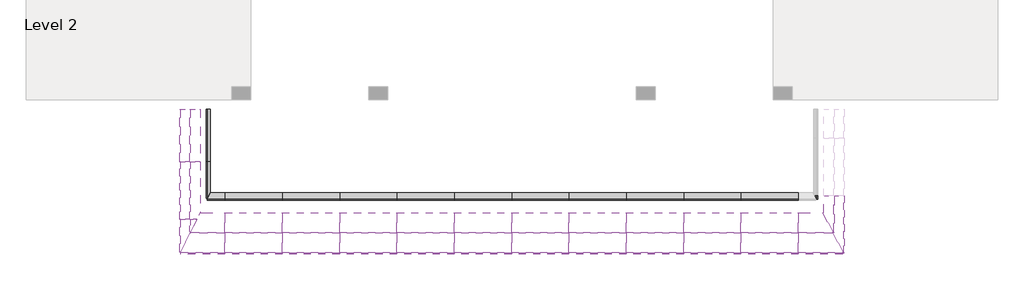
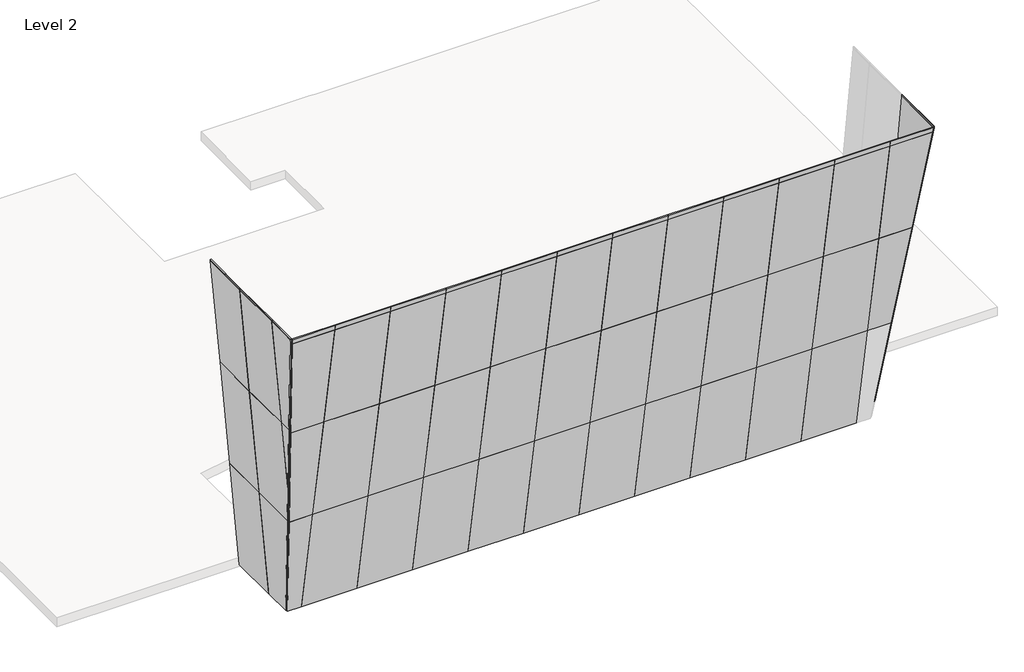
# One storey, part 1 of 2: 62 plates.
"""IFC4 building model written with IfcOpenShell, lengths in millimetres."""

import ifcopenshell
import ifcopenshell.guid

model = None  # the IFC model being written
_history = None  # IfcOwnerHistory: only IFC2X3 demands one
_inside = {}  # id of a spatial element -> (the spatial element, [elements in it])
_under = {}  # id of a project, library or spatial element -> (it, [spatial elements below it])
_declared = {}  # id of a project -> (the project, [libraries it declares])
_typed = {}  # id of a type object -> (the type object, [elements of that type])
_made_of = {}  # id of a material, layer set ... -> (it, [elements and type objects made of it])


def new_model(schema):
    """Start an empty IFC model of exactly this schema.

    Asked for "IFC4X3", IfcOpenShell would pick the latest addendum, in which some entities
    have other attributes; the version numbers below select the first issue.
    IFC2X3 requires an IfcOwnerHistory on every rooted entity: one is made here for all.
    """
    global model, _history
    if schema == "IFC4X3":
        model = ifcopenshell.file(schema_version=(4, 3, 0, 0))
    else:
        model = ifcopenshell.file(schema=schema)
    _inside.clear()
    _under.clear()
    _declared.clear()
    _typed.clear()
    _made_of.clear()
    _history = None
    if model.schema == "IFC2X3":
        org = make("IfcOrganization", Name="unknown")
        user = make(
            "IfcPersonAndOrganization",
            ThePerson=make("IfcPerson", FamilyName="unknown"),
            TheOrganization=org,
        )
        app = make(
            "IfcApplication",
            ApplicationDeveloper=org,
            Version="unknown",
            ApplicationFullName="unknown",
            ApplicationIdentifier="unknown",
        )
        _history = make(
            "IfcOwnerHistory",
            OwningUser=user,
            OwningApplication=app,
            ChangeAction="ADDED",
            CreationDate=0,
        )
    return model


def make(cls, **values):
    """One entity of the class cls with the attributes given. An attribute that is None is left unset."""
    return model.create_entity(
        cls, **{name: value for name, value in values.items() if value is not None}
    )


def rooted(cls, **values):
    """An entity with a GlobalId (a new one), such as an element, a storey or a relation."""
    return make(cls, GlobalId=ifcopenshell.guid.new(), OwnerHistory=_history, **values)


def si_unit(unit_type, name, prefix=None):
    """IfcSIUnit, for example si_unit("LENGTHUNIT", "METRE", prefix="MILLI")."""
    return make("IfcSIUnit", UnitType=unit_type, Prefix=prefix, Name=name)


def assignment(units):
    """IfcUnitAssignment: the units of a project."""
    return None if units is None else make("IfcUnitAssignment", Units=units)


def point(xyz):
    """IfcCartesianPoint."""
    return None if xyz is None else make("IfcCartesianPoint", Coordinates=xyz)


def direction(xyz):
    """IfcDirection."""
    return None if xyz is None else make("IfcDirection", DirectionRatios=xyz)


def frame(location, z_axis=None, x_axis=None):
    """IfcAxis2Placement3D, a coordinate frame: its origin and axes. An axis left out is left unset."""
    return make(
        "IfcAxis2Placement3D",
        Location=point(location),
        Axis=direction(z_axis),
        RefDirection=direction(x_axis),
    )


def origin():
    """The frame at (0, 0, 0) with its axes left unset."""
    return frame((0.0, 0.0, 0.0))


def origin_with_axes():
    """The frame at (0, 0, 0) with the z axis (0, 0, 1) and the x axis (1, 0, 0) written out."""
    return frame((0.0, 0.0, 0.0), z_axis=(0.0, 0.0, 1.0), x_axis=(1.0, 0.0, 0.0))


def place(relative_to, where):
    """IfcLocalPlacement: puts the frame where relative to a parent placement (None: the world)."""
    return make(
        "IfcLocalPlacement", PlacementRelTo=relative_to, RelativePlacement=where
    )


def context(
    kind, dimensions, precision=None, world=None, true_north=None, identifier=None
):
    """IfcGeometricRepresentationContext, for example the 3D "Model" context."""
    return make(
        "IfcGeometricRepresentationContext",
        ContextIdentifier=identifier,
        ContextType=kind,
        CoordinateSpaceDimension=dimensions,
        Precision=precision,
        WorldCoordinateSystem=world,
        TrueNorth=true_north,
    )


def project(units=None, contexts=None):
    """IfcProject with its units and contexts."""
    return rooted(
        "IfcProject",
        Name="project",
        RepresentationContexts=contexts,
        UnitsInContext=assignment(units),
    )


def spatial(cls, under=None, at=None, **own):
    """A site, building, storey or space (cls), placed at a placement, below another one or the project."""
    s = rooted(cls, ObjectPlacement=at, **own)
    if under is not None:
        _under.setdefault(under.id(), (under, []))[1].append(s)
    return s


def polyline(points):
    """IfcPolyline through the points."""
    return make("IfcPolyline", Points=[point(p) for p in points])


def outline(outer, holes=None, kind="AREA"):
    """IfcArbitraryClosedProfileDef: a profile drawn as a closed curve; with holes, ...WithVoids."""
    if holes is None:
        return make("IfcArbitraryClosedProfileDef", ProfileType=kind, OuterCurve=outer)
    return make(
        "IfcArbitraryProfileDefWithVoids",
        ProfileType=kind,
        OuterCurve=outer,
        InnerCurves=holes,
    )


def extrude(swept, where, along, depth):
    """IfcExtrudedAreaSolid: the profile swept, set in the frame where, extruded along a direction by depth."""
    return make(
        "IfcExtrudedAreaSolid",
        SweptArea=swept,
        Position=where,
        ExtrudedDirection=direction(along),
        Depth=depth,
    )


def shape(context_of_items, identifier, shape_type, items):
    """IfcShapeRepresentation: the items that make up one representation, for example the "Body"."""
    return make(
        "IfcShapeRepresentation",
        ContextOfItems=context_of_items,
        RepresentationIdentifier=identifier,
        RepresentationType=shape_type,
        Items=items,
    )


def source(mapping_origin, context_of_items, identifier, shape_type, items):
    """IfcRepresentationMap: a shape defined once, which mapped items show again and again."""
    return make(
        "IfcRepresentationMap",
        MappingOrigin=mapping_origin,
        MappedRepresentation=shape(context_of_items, identifier, shape_type, items),
    )


def transform(
    local_origin,
    x_axis=None,
    y_axis=None,
    z_axis=None,
    scale=None,
    scale2=None,
    scale3=None,
    uniform=True,
):
    """IfcCartesianTransformationOperator3D, or its non-uniform kind. x_axis, y_axis, z_axis: its Axis1, 2, 3."""
    if uniform:
        return make(
            "IfcCartesianTransformationOperator3D",
            Axis1=direction(x_axis),
            Axis2=direction(y_axis),
            LocalOrigin=point(local_origin),
            Scale=scale,
            Axis3=direction(z_axis),
        )
    return make(
        "IfcCartesianTransformationOperator3DnonUniform",
        Axis1=direction(x_axis),
        Axis2=direction(y_axis),
        LocalOrigin=point(local_origin),
        Scale=scale,
        Axis3=direction(z_axis),
        Scale2=scale2,
        Scale3=scale3,
    )


def mapped(mapping_source, mapping_target):
    """IfcMappedItem: shows the shape of a source again, moved by a transform."""
    return make(
        "IfcMappedItem", MappingSource=mapping_source, MappingTarget=mapping_target
    )


def made_of(thing, what):
    """Note that an element or type object is made of a material, layer set ...; save() writes the relation."""
    if what is not None:
        _made_of.setdefault(what.id(), (what, []))[1].append(thing)
    return thing


def element(
    cls,
    number,
    at=None,
    inside=None,
    cuts=None,
    type_object=None,
    material=None,
    context=None,
    identifier="Body",
    shape_type=None,
    held_by="IfcProductDefinitionShape",
    body=None,
    shapes=None,
    **own,
):
    """One element of the class cls, such as IfcWall. Its Tag is "e" and its number.

    at: its placement. inside: the storey or other place that contains it. cuts: it is an
    opening in that element (IfcRelVoidsElement). A single representation is given by context,
    identifier, shape_type and body (its items); several are given by shapes. held_by: the class
    of the entity that holds the representations. save() writes the other relations.
    """
    e = rooted(cls, Tag="e%d" % number, ObjectPlacement=at, **own)
    if body is not None:
        shapes = [shape(context, identifier, shape_type, body)]
    if shapes is not None:
        e.Representation = make(held_by, Representations=shapes)
    if inside is not None:
        _inside.setdefault(inside.id(), (inside, []))[1].append(e)
    if cuts is not None:
        rooted(
            "IfcRelVoidsElement", RelatingBuildingElement=cuts, RelatedOpeningElement=e
        )
    if type_object is not None:
        _typed.setdefault(type_object.id(), (type_object, []))[1].append(e)
    return made_of(e, material)


def aggregate(whole, parts):
    """IfcRelAggregates: a whole, such as a stair, and the parts it consists of."""
    return rooted("IfcRelAggregates", RelatingObject=whole, RelatedObjects=parts)


def save(model, path):
    """Write the relations noted so far, then the file.

    IfcRelAggregates (storeys below a building ...), IfcRelContainedInSpatialStructure (elements
    in a storey), IfcRelDefinesByType, IfcRelAssociatesMaterial and IfcRelDeclares: one each for
    every whole, place, type object, material and project.
    """
    for whole, parts in _under.values():
        aggregate(whole, parts)
    for where, things in _inside.values():
        rooted(
            "IfcRelContainedInSpatialStructure",
            RelatedElements=things,
            RelatingStructure=where,
        )
    for kind, things in _typed.values():
        rooted("IfcRelDefinesByType", RelatedObjects=things, RelatingType=kind)
    for what, things in _made_of.values():
        rooted("IfcRelAssociatesMaterial", RelatedObjects=things, RelatingMaterial=what)
    for by, libraries in _declared.values():
        rooted("IfcRelDeclares", RelatingContext=by, RelatedDefinitions=libraries)
    model.write(path)


def system_panel_glazed_2e91cb65(model_context):
    return source(origin(), model_context, "Body", "SweptSolid", [
        extrude(outline(polyline([(838.2000002, -44.45), (-838.2000002, -44.45), (-838.2000002, -19.05), (838.2000002, -19.05), (838.2000002, -44.45)])), origin_with_axes(), (0.0, 0.0, 1.0), 3657.6),
    ])


def system_panel_glazed_41c8569a(model_context):
    return source(origin(), model_context, "Body", "SweptSolid", [
        extrude(outline(polyline([(3054.1438606, -268.2393521), (0.0, 268.2393521), (3054.1438606, 268.2393521), (3054.1438606, -268.2393521)])), frame((0.0, -44.45, 0.0), z_axis=(0.0, 1.0, 0.0), x_axis=(0.0, 0.0, 1.0)), (0.0, 0.0, 1.0), 25.4),
    ])


def system_panel_glazed_2bad594a(model_context):
    return source(origin(), model_context, "Body", "SweptSolid", [
        extrude(outline(polyline([(0.0, -797.3917397), (0.0, 154.912342), (3657.6, 797.3917397), (3657.6, -797.3917397), (0.0, -797.3917397)])), frame((0.0, -44.45, 0.0), z_axis=(0.0, 1.0, 0.0), x_axis=(0.0, 0.0, 1.0)), (0.0, 0.0, 1.0), 25.4),
    ])


def system_panel_glazed_87679f4c(model_context):
    return source(origin(), model_context, "Body", "SweptSolid", [
        extrude(outline(polyline([(0.0, -914.4), (0.0, 680.3834794), (1332.2432262, 914.4), (3657.6, 914.4), (3657.6, -914.4), (0.0, -914.4)])), frame((0.0, -44.45, 0.0), z_axis=(0.0, 1.0, 0.0), x_axis=(0.0, 0.0, 1.0)), (0.0, 0.0, 1.0), 25.4),
    ])


def system_panel_glazed_96c5221b(model_context):
    return source(origin(), model_context, "Body", "SweptSolid", [
        extrude(outline(polyline([(0.0, -204.2314386), (2325.3567738, 204.2314386), (2325.3567738, -204.2314386), (0.0, -204.2314386)])), frame((0.0, -44.45, 0.0), z_axis=(0.0, 1.0, 0.0), x_axis=(0.0, 0.0, 1.0)), (0.0, 0.0, 1.0), 25.4),
    ])


def system_panel_glazed_1f34555f(model_context):
    return source(origin(), model_context, "Body", "SweptSolid", [
        extrude(outline(polyline([(914.4, -44.45), (-914.4, -44.45), (-914.4, -19.05), (914.4, -19.05), (914.4, -44.45)])), origin_with_axes(), (0.0, 0.0, 1.0), 3657.6),
    ])


def system_panel_glazed_ce152239(model_context):
    return source(origin(), model_context, "Body", "SweptSolid", [
        extrude(outline(polyline([(0.0, -525.4711374), (0.0, -117.0082603), (3657.6, 525.4711374), (3657.6, -525.4711374), (0.0, -525.4711374)])), frame((0.0, -44.45, 0.0), z_axis=(0.0, 1.0, 0.0), x_axis=(0.0, 0.0, 1.0)), (0.0, 0.0, 1.0), 25.4),
    ])


def system_panel_glazed_8b4ddac8(model_context):
    return source(origin(), model_context, "Body", "SweptSolid", [
        extrude(outline(polyline([(838.2000002, -44.45), (-838.2000002, -44.45), (-838.2000002, -19.05), (838.2000002, -19.05), (838.2000002, -44.45)])), origin_with_axes(), (0.0, 0.0, 1.0), 41.9143134),
    ])


def system_panel_glazed_7f82afe2(model_context):
    return source(origin(), model_context, "Body", "SweptSolid", [
        extrude(outline(polyline([(914.4, -44.45), (-914.4, -44.45), (-914.4, -19.05), (914.4, -19.05), (914.4, -44.45)])), origin_with_axes(), (0.0, 0.0, 1.0), 41.9143134),
    ])


def system_panel_glazed_3146f186(model_context):
    return source(origin(), model_context, "Body", "SweptSolid", [
        extrude(outline(polyline([(0.0, -529.1523878), (0.0, 521.789887), (41.9143134, 529.1523878), (41.9143134, -529.1523878), (0.0, -529.1523878)])), frame((0.0, -44.45, 0.0), z_axis=(0.0, 1.0, 0.0), x_axis=(0.0, 0.0, 1.0)), (0.0, 0.0, 1.0), 25.4),
    ])


def system_panel_glazed_f4345ae3(model_context):
    return source(origin(), model_context, "Body", "SweptSolid", [
        extrude(outline(polyline([(914.4, -44.45), (-914.4, -44.45), (-914.4, -19.05), (914.4, -19.05), (914.4, -44.45)])), origin_with_axes(), (0.0, 0.0, 1.0), 169.2731269),
    ])


def system_panel_glazed_bcd6892e(model_context):
    return source(origin(), model_context, "Body", "SweptSolid", [
        extrude(outline(polyline([(0.0, 53.0003468), (0.0, 589.4790509), (3657.6, 589.4790509), (3657.6, -589.4790509), (0.0, 53.0003468)])), frame((0.0, -44.45, 0.0), z_axis=(0.0, 1.0, 0.0), x_axis=(0.0, 0.0, 1.0)), (0.0, 0.0, 1.0), 25.4),
    ])


def system_panel_glazed_e7bd2299(model_context):
    return source(origin(), model_context, "Body", "SweptSolid", [
        extrude(outline(polyline([(0.0, -268.2393521), (0.0, 910.7187498), (3657.6, 910.7187498), (3657.6, -910.7187498), (0.0, -268.2393521)])), frame((0.0, -44.45, 0.0), z_axis=(0.0, 1.0, 0.0), x_axis=(0.0, 0.0, 1.0)), (0.0, 0.0, 1.0), 25.4),
    ])


def system_panel_glazed_0a43eb3e(model_context):
    return source(origin(), model_context, "Body", "SweptSolid", [
        extrude(outline(polyline([(0.0, -907.0374994), (0.0, 914.4000002), (41.9143134, 914.4000002), (41.9143134, -914.4000002), (0.0, -907.0374994)])), frame((0.0, -44.45, 0.0), z_axis=(0.0, 1.0, 0.0), x_axis=(0.0, 0.0, 1.0)), (0.0, 0.0, 1.0), 25.4),
    ])


def system_panel_glazed_35afb83b(model_context):
    return source(origin(), model_context, "Body", "SweptSolid", [
        extrude(outline(polyline([(0.0, -71.0314805), (0.0, 386.1685195), (3657.6, 386.1685195), (3657.6, -386.1685195), (0.0, -71.0314805)])), frame((0.0, -44.45, 0.0), z_axis=(0.0, 1.0, 0.0), x_axis=(0.0, 0.0, 1.0)), (0.0, 0.0, 1.0), 25.4),
    ])


def system_panel_glazed_d5b9b34d(model_context):
    return source(origin(), model_context, "Body", "SweptSolid", [
        extrude(outline(polyline([(0.0, -228.6), (0.0, 543.7370389), (3657.6, 543.7370389), (3657.6, -543.7370389), (0.0, -228.6)])), frame((0.0, -44.45, 0.0), z_axis=(0.0, 1.0, 0.0), x_axis=(0.0, 0.0, 1.0)), (0.0, 0.0, 1.0), 25.4),
    ])


def system_panel_glazed_127879aa(model_context):
    return source(origin(), model_context, "Body", "SweptSolid", [
        extrude(outline(polyline([(0.0, -543.7370389), (0.0, 228.6), (3657.6, 543.7370389), (3657.6, -543.7370389), (0.0, -543.7370389)])), frame((0.0, -44.45, 0.0), z_axis=(0.0, 1.0, 0.0), x_axis=(0.0, 0.0, 1.0)), (0.0, 0.0, 1.0), 25.4),
    ])


def system_panel_glazed_cde5e94a(model_context):
    return source(origin(), model_context, "Body", "SweptSolid", [
        extrude(outline(polyline([(0.0, -386.1685195), (0.0, 701.3055584), (3657.6, 701.3055584), (3657.6, -701.3055584), (0.0, -386.1685195)])), frame((0.0, -44.45, 0.0), z_axis=(0.0, 1.0, 0.0), x_axis=(0.0, 0.0, 1.0)), (0.0, 0.0, 1.0), 25.4),
    ])


def system_panel_glazed_b3fa7013(model_context):
    return source(origin(), model_context, "Body", "SweptSolid", [
        extrude(outline(polyline([(0.0, -701.3055584), (0.0, 386.1685195), (3657.6, 701.3055584), (3657.6, -701.3055584), (0.0, -701.3055584)])), frame((0.0, -44.45, 0.0), z_axis=(0.0, 1.0, 0.0), x_axis=(0.0, 0.0, 1.0)), (0.0, 0.0, 1.0), 25.4),
    ])


def system_panel_glazed_d86b06c2(model_context):
    return source(origin(), model_context, "Body", "SweptSolid", [
        extrude(outline(polyline([(0.0, -694.0133132), (0.0, 708.5978036), (169.2731269, 708.5978036), (169.2731269, -708.5978036), (0.0, -694.0133132)])), frame((0.0, -44.45, 0.0), z_axis=(0.0, 1.0, 0.0), x_axis=(0.0, 0.0, 1.0)), (0.0, 0.0, 1.0), 25.4),
    ])


def system_panel_glazed_9c30f1a4(model_context):
    return source(origin(), model_context, "Body", "SweptSolid", [
        extrude(outline(polyline([(0.0, -708.5978036), (0.0, 694.0133132), (169.2731269, 708.5978036), (169.2731269, -708.5978036), (0.0, -708.5978036)])), frame((0.0, -44.45, 0.0), z_axis=(0.0, 1.0, 0.0), x_axis=(0.0, 0.0, 1.0)), (0.0, 0.0, 1.0), 25.4),
    ])


model = new_model("IFC4")

# Units and contexts
model_context = context("Model", 3, world=origin())
ifc_project = project(units=[si_unit("LENGTHUNIT", "METRE", prefix="MILLI")], contexts=[model_context])

# Site, building, storey
site = spatial("IfcSite", under=ifc_project)
building = spatial("IfcBuilding", under=site)
storey = spatial("IfcBuildingStorey", under=building, Name="Level 2", Elevation=3657.6)

# Plates
placement = place(None, origin())
system_panel_glazed_shape = system_panel_glazed_2e91cb65(model_context)
element("IfcPlate", 1, ObjectType="System Panel : Glazed", at=placement, inside=storey, context=model_context, shape_type="MappedRepresentation", body=[
    mapped(system_panel_glazed_shape, transform((-10766.9154339, -10749.0984697, 3656.4931221), x_axis=(0.0, -1.0, 0.0), y_axis=(0.9961946980917455, 0.0, 0.08715574274765803), z_axis=(-0.08715574274765803, 0.0, 0.9961946980917455))),
])
element("IfcPlate", 2, ObjectType="System Panel : Glazed", at=placement, inside=storey, context=model_context, shape_type="MappedRepresentation", body=[
    mapped(system_panel_glazed_shape, transform((-11085.6962786, -10749.0984697, 7300.1748498), x_axis=(0.0, -1.0, 0.0), y_axis=(0.9961946980917455, 0.0, 0.08715574274765803), z_axis=(-0.08715574274765803, 0.0, 0.9961946980917455))),
])
element("IfcPlate", 3, ObjectType="System Panel : Glazed", at=placement, inside=storey, context=model_context, shape_type="MappedRepresentation", body=[
    mapped(system_panel_glazed_shape, transform((-11404.4771233, -10749.0984697, 10943.8565775), x_axis=(0.0, -1.0, 0.0), y_axis=(0.9961946980917455, 0.0, 0.08715574274765803), z_axis=(-0.08715574274765803, 0.0, 0.9961946980917455))),
])
system_panel_glazed_2_shape = system_panel_glazed_41c8569a(model_context)
element("IfcPlate", 4, ObjectType="System Panel : Glazed", at=placement, inside=storey, context=model_context, shape_type="MappedRepresentation", body=[
    mapped(system_panel_glazed_2_shape, transform((8487.8855556, -12939.6344332, 4257.6529286), x_axis=(0.0, 1.0, 0.0), y_axis=(-0.9961946980917455, 0.0, 0.08715574274765803), z_axis=(0.08715574274765803, 0.0, 0.9961946980917455))),
])
system_panel_glazed_3_shape = system_panel_glazed_2bad594a(model_context)
element("IfcPlate", 5, ObjectType="System Panel : Glazed", at=placement, inside=storey, context=model_context, shape_type="MappedRepresentation", body=[
    mapped(system_panel_glazed_3_shape, transform((-10766.9154339, -12384.6902096, 3656.4931221), x_axis=(0.0, -1.0, 0.0), y_axis=(0.9961946980917455, 0.0, 0.08715574274765803), z_axis=(-0.08715574274765803, 0.0, 0.9961946980917455))),
])
system_panel_glazed_4_shape = system_panel_glazed_87679f4c(model_context)
element("IfcPlate", 6, ObjectType="System Panel : Glazed", at=placement, inside=storey, context=model_context, shape_type="MappedRepresentation", body=[
    mapped(system_panel_glazed_4_shape, transform((-11085.6962786, -12501.6984699, 7300.1748498), x_axis=(0.0, -1.0, 0.0), y_axis=(0.9961946980917455, 0.0, 0.08715574274765803), z_axis=(-0.08715574274765803, 0.0, 0.9961946980917455))),
])
system_panel_glazed_5_shape = system_panel_glazed_96c5221b(model_context)
element("IfcPlate", 7, ObjectType="System Panel : Glazed", at=placement, inside=storey, context=model_context, shape_type="MappedRepresentation", body=[
    mapped(system_panel_glazed_5_shape, transform((-11201.8089265, -13620.3299085, 8627.3484884), x_axis=(0.0, -1.0, 0.0), y_axis=(0.9961946980917455, 0.0, 0.08715574274765803), z_axis=(-0.08715574274765803, 0.0, 0.9961946980917455))),
])
system_panel_glazed_6_shape = system_panel_glazed_1f34555f(model_context)
element("IfcPlate", 8, ObjectType="System Panel : Glazed", at=placement, inside=storey, context=model_context, shape_type="MappedRepresentation", body=[
    mapped(system_panel_glazed_6_shape, transform((-11404.4771233, -12501.6984699, 10943.8565775), x_axis=(0.0, -1.0, 0.0), y_axis=(0.9961946980917455, 0.0, 0.08715574274765803), z_axis=(-0.08715574274765803, 0.0, 0.9961946980917455))),
])
element("IfcPlate", 9, ObjectType="System Panel : Glazed", at=placement, inside=storey, context=model_context, shape_type="MappedRepresentation", body=[
    mapped(system_panel_glazed_6_shape, transform((-9408.1607851, -12552.1096101, 3655.3946681), x_axis=(1.0, 0.0, 0.0), y_axis=(0.0, 0.9848077530122081, 0.17364817766693014), z_axis=(0.0, -0.17364817766693014, 0.9848077530122081))),
])
element("IfcPlate", 10, ObjectType="System Panel : Glazed", at=placement, inside=storey, context=model_context, shape_type="MappedRepresentation", body=[
    mapped(system_panel_glazed_6_shape, transform((-7579.3607851, -12552.1096101, 3655.3946681), x_axis=(1.0, 0.0, 0.0), y_axis=(0.0, 0.9848077530122081, 0.17364817766693014), z_axis=(0.0, -0.17364817766693014, 0.9848077530122081))),
])
element("IfcPlate", 11, ObjectType="System Panel : Glazed", at=placement, inside=storey, context=model_context, shape_type="MappedRepresentation", body=[
    mapped(system_panel_glazed_6_shape, transform((-5750.5607851, -12552.1096101, 3655.3946681), x_axis=(1.0, 0.0, 0.0), y_axis=(0.0, 0.9848077530122081, 0.17364817766693014), z_axis=(0.0, -0.17364817766693014, 0.9848077530122081))),
])
element("IfcPlate", 12, ObjectType="System Panel : Glazed", at=placement, inside=storey, context=model_context, shape_type="MappedRepresentation", body=[
    mapped(system_panel_glazed_6_shape, transform((-3921.7607851, -12552.1096101, 3655.3946681), x_axis=(1.0, 0.0, 0.0), y_axis=(0.0, 0.9848077530122081, 0.17364817766693014), z_axis=(0.0, -0.17364817766693014, 0.9848077530122081))),
])
element("IfcPlate", 13, ObjectType="System Panel : Glazed", at=placement, inside=storey, context=model_context, shape_type="MappedRepresentation", body=[
    mapped(system_panel_glazed_6_shape, transform((-2092.9607851, -12552.1096101, 3655.3946681), x_axis=(1.0, 0.0, 0.0), y_axis=(0.0, 0.9848077530122081, 0.17364817766693014), z_axis=(0.0, -0.17364817766693014, 0.9848077530122081))),
])
element("IfcPlate", 14, ObjectType="System Panel : Glazed", at=placement, inside=storey, context=model_context, shape_type="MappedRepresentation", body=[
    mapped(system_panel_glazed_6_shape, transform((-264.1607851, -12552.1096101, 3655.3946681), x_axis=(1.0, 0.0, 0.0), y_axis=(0.0, 0.9848077530122081, 0.17364817766693014), z_axis=(0.0, -0.17364817766693014, 0.9848077530122081))),
])
element("IfcPlate", 15, ObjectType="System Panel : Glazed", at=placement, inside=storey, context=model_context, shape_type="MappedRepresentation", body=[
    mapped(system_panel_glazed_6_shape, transform((1564.6392149, -12552.1096101, 3655.3946681), x_axis=(1.0, 0.0, 0.0), y_axis=(0.0, 0.9848077530122081, 0.17364817766693014), z_axis=(0.0, -0.17364817766693014, 0.9848077530122081))),
])
element("IfcPlate", 16, ObjectType="System Panel : Glazed", at=placement, inside=storey, context=model_context, shape_type="MappedRepresentation", body=[
    mapped(system_panel_glazed_6_shape, transform((3393.4392149, -12552.1096101, 3655.3946681), x_axis=(1.0, 0.0, 0.0), y_axis=(0.0, 0.9848077530122081, 0.17364817766693014), z_axis=(0.0, -0.17364817766693014, 0.9848077530122081))),
])
element("IfcPlate", 17, ObjectType="System Panel : Glazed", at=placement, inside=storey, context=model_context, shape_type="MappedRepresentation", body=[
    mapped(system_panel_glazed_6_shape, transform((5222.2392149, -12552.1096101, 3655.3946681), x_axis=(1.0, 0.0, 0.0), y_axis=(0.0, 0.9848077530122081, 0.17364817766693014), z_axis=(0.0, -0.17364817766693014, 0.9848077530122081))),
])
element("IfcPlate", 18, ObjectType="System Panel : Glazed", at=placement, inside=storey, context=model_context, shape_type="MappedRepresentation", body=[
    mapped(system_panel_glazed_6_shape, transform((7051.0392149, -12552.1096101, 3655.3946681), x_axis=(1.0, 0.0, 0.0), y_axis=(0.0, 0.9848077530122081, 0.17364817766693014), z_axis=(0.0, -0.17364817766693014, 0.9848077530122081))),
])
element("IfcPlate", 19, ObjectType="System Panel : Glazed", at=placement, inside=storey, context=model_context, shape_type="MappedRepresentation", body=[
    mapped(system_panel_glazed_6_shape, transform((-9408.1607851, -13187.2451847, 7257.4275056), x_axis=(1.0, 0.0, 0.0), y_axis=(0.0, 0.9848077530122081, 0.17364817766693014), z_axis=(0.0, -0.17364817766693014, 0.9848077530122081))),
])
element("IfcPlate", 20, ObjectType="System Panel : Glazed", at=placement, inside=storey, context=model_context, shape_type="MappedRepresentation", body=[
    mapped(system_panel_glazed_6_shape, transform((-7579.3607851, -13187.2451847, 7257.4275056), x_axis=(1.0, 0.0, 0.0), y_axis=(0.0, 0.9848077530122081, 0.17364817766693014), z_axis=(0.0, -0.17364817766693014, 0.9848077530122081))),
])
element("IfcPlate", 21, ObjectType="System Panel : Glazed", at=placement, inside=storey, context=model_context, shape_type="MappedRepresentation", body=[
    mapped(system_panel_glazed_6_shape, transform((-5750.5607851, -13187.2451847, 7257.4275056), x_axis=(1.0, 0.0, 0.0), y_axis=(0.0, 0.9848077530122081, 0.17364817766693014), z_axis=(0.0, -0.17364817766693014, 0.9848077530122081))),
])
element("IfcPlate", 22, ObjectType="System Panel : Glazed", at=placement, inside=storey, context=model_context, shape_type="MappedRepresentation", body=[
    mapped(system_panel_glazed_6_shape, transform((-3921.7607851, -13187.2451847, 7257.4275056), x_axis=(1.0, 0.0, 0.0), y_axis=(0.0, 0.9848077530122081, 0.17364817766693014), z_axis=(0.0, -0.17364817766693014, 0.9848077530122081))),
])
element("IfcPlate", 23, ObjectType="System Panel : Glazed", at=placement, inside=storey, context=model_context, shape_type="MappedRepresentation", body=[
    mapped(system_panel_glazed_6_shape, transform((-2092.9607851, -13187.2451847, 7257.4275056), x_axis=(1.0, 0.0, 0.0), y_axis=(0.0, 0.9848077530122081, 0.17364817766693014), z_axis=(0.0, -0.17364817766693014, 0.9848077530122081))),
])
element("IfcPlate", 24, ObjectType="System Panel : Glazed", at=placement, inside=storey, context=model_context, shape_type="MappedRepresentation", body=[
    mapped(system_panel_glazed_6_shape, transform((-264.1607851, -13187.2451847, 7257.4275056), x_axis=(1.0, 0.0, 0.0), y_axis=(0.0, 0.9848077530122081, 0.17364817766693014), z_axis=(0.0, -0.17364817766693014, 0.9848077530122081))),
])
element("IfcPlate", 25, ObjectType="System Panel : Glazed", at=placement, inside=storey, context=model_context, shape_type="MappedRepresentation", body=[
    mapped(system_panel_glazed_6_shape, transform((1564.6392149, -13187.2451847, 7257.4275056), x_axis=(1.0, 0.0, 0.0), y_axis=(0.0, 0.9848077530122081, 0.17364817766693014), z_axis=(0.0, -0.17364817766693014, 0.9848077530122081))),
])
element("IfcPlate", 26, ObjectType="System Panel : Glazed", at=placement, inside=storey, context=model_context, shape_type="MappedRepresentation", body=[
    mapped(system_panel_glazed_6_shape, transform((3393.4392149, -13187.2451847, 7257.4275056), x_axis=(1.0, 0.0, 0.0), y_axis=(0.0, 0.9848077530122081, 0.17364817766693014), z_axis=(0.0, -0.17364817766693014, 0.9848077530122081))),
])
element("IfcPlate", 27, ObjectType="System Panel : Glazed", at=placement, inside=storey, context=model_context, shape_type="MappedRepresentation", body=[
    mapped(system_panel_glazed_6_shape, transform((5222.2392149, -13187.2451847, 7257.4275056), x_axis=(1.0, 0.0, 0.0), y_axis=(0.0, 0.9848077530122081, 0.17364817766693014), z_axis=(0.0, -0.17364817766693014, 0.9848077530122081))),
])
element("IfcPlate", 28, ObjectType="System Panel : Glazed", at=placement, inside=storey, context=model_context, shape_type="MappedRepresentation", body=[
    mapped(system_panel_glazed_6_shape, transform((7051.0392149, -13187.2451847, 7257.4275056), x_axis=(1.0, 0.0, 0.0), y_axis=(0.0, 0.9848077530122081, 0.17364817766693014), z_axis=(0.0, -0.17364817766693014, 0.9848077530122081))),
])
element("IfcPlate", 29, ObjectType="System Panel : Glazed", at=placement, inside=storey, context=model_context, shape_type="MappedRepresentation", body=[
    mapped(system_panel_glazed_6_shape, transform((-9408.1607851, -13822.3807593, 10859.460343), x_axis=(1.0, 0.0, 0.0), y_axis=(0.0, 0.9848077530122081, 0.17364817766693014), z_axis=(0.0, -0.17364817766693014, 0.9848077530122081))),
])
element("IfcPlate", 30, ObjectType="System Panel : Glazed", at=placement, inside=storey, context=model_context, shape_type="MappedRepresentation", body=[
    mapped(system_panel_glazed_6_shape, transform((-7579.3607851, -13822.3807593, 10859.460343), x_axis=(1.0, 0.0, 0.0), y_axis=(0.0, 0.9848077530122081, 0.17364817766693014), z_axis=(0.0, -0.17364817766693014, 0.9848077530122081))),
])
element("IfcPlate", 31, ObjectType="System Panel : Glazed", at=placement, inside=storey, context=model_context, shape_type="MappedRepresentation", body=[
    mapped(system_panel_glazed_6_shape, transform((-5750.5607851, -13822.3807593, 10859.460343), x_axis=(1.0, 0.0, 0.0), y_axis=(0.0, 0.9848077530122081, 0.17364817766693014), z_axis=(0.0, -0.17364817766693014, 0.9848077530122081))),
])
element("IfcPlate", 32, ObjectType="System Panel : Glazed", at=placement, inside=storey, context=model_context, shape_type="MappedRepresentation", body=[
    mapped(system_panel_glazed_6_shape, transform((-3921.7607851, -13822.3807593, 10859.460343), x_axis=(1.0, 0.0, 0.0), y_axis=(0.0, 0.9848077530122081, 0.17364817766693014), z_axis=(0.0, -0.17364817766693014, 0.9848077530122081))),
])
element("IfcPlate", 33, ObjectType="System Panel : Glazed", at=placement, inside=storey, context=model_context, shape_type="MappedRepresentation", body=[
    mapped(system_panel_glazed_6_shape, transform((-2092.9607851, -13822.3807593, 10859.460343), x_axis=(1.0, 0.0, 0.0), y_axis=(0.0, 0.9848077530122081, 0.17364817766693014), z_axis=(0.0, -0.17364817766693014, 0.9848077530122081))),
])
element("IfcPlate", 34, ObjectType="System Panel : Glazed", at=placement, inside=storey, context=model_context, shape_type="MappedRepresentation", body=[
    mapped(system_panel_glazed_6_shape, transform((-264.1607851, -13822.3807593, 10859.460343), x_axis=(1.0, 0.0, 0.0), y_axis=(0.0, 0.9848077530122081, 0.17364817766693014), z_axis=(0.0, -0.17364817766693014, 0.9848077530122081))),
])
element("IfcPlate", 35, ObjectType="System Panel : Glazed", at=placement, inside=storey, context=model_context, shape_type="MappedRepresentation", body=[
    mapped(system_panel_glazed_6_shape, transform((1564.6392149, -13822.3807593, 10859.460343), x_axis=(1.0, 0.0, 0.0), y_axis=(0.0, 0.9848077530122081, 0.17364817766693014), z_axis=(0.0, -0.17364817766693014, 0.9848077530122081))),
])
element("IfcPlate", 36, ObjectType="System Panel : Glazed", at=placement, inside=storey, context=model_context, shape_type="MappedRepresentation", body=[
    mapped(system_panel_glazed_6_shape, transform((3393.4392149, -13822.3807593, 10859.460343), x_axis=(1.0, 0.0, 0.0), y_axis=(0.0, 0.9848077530122081, 0.17364817766693014), z_axis=(0.0, -0.17364817766693014, 0.9848077530122081))),
])
element("IfcPlate", 37, ObjectType="System Panel : Glazed", at=placement, inside=storey, context=model_context, shape_type="MappedRepresentation", body=[
    mapped(system_panel_glazed_6_shape, transform((5222.2392149, -13822.3807593, 10859.460343), x_axis=(1.0, 0.0, 0.0), y_axis=(0.0, 0.9848077530122081, 0.17364817766693014), z_axis=(0.0, -0.17364817766693014, 0.9848077530122081))),
])
element("IfcPlate", 38, ObjectType="System Panel : Glazed", at=placement, inside=storey, context=model_context, shape_type="MappedRepresentation", body=[
    mapped(system_panel_glazed_6_shape, transform((7051.0392149, -13822.3807593, 10859.460343), x_axis=(1.0, 0.0, 0.0), y_axis=(0.0, 0.9848077530122081, 0.17364817766693014), z_axis=(0.0, -0.17364817766693014, 0.9848077530122081))),
])
system_panel_glazed_7_shape = system_panel_glazed_ce152239(model_context)
element("IfcPlate", 39, ObjectType="System Panel : Glazed", at=placement, inside=storey, context=model_context, shape_type="MappedRepresentation", body=[
    mapped(system_panel_glazed_7_shape, transform((-11404.4771233, -13941.5696073, 10943.8565775), x_axis=(0.0, -1.0, 0.0), y_axis=(0.9961946980917455, 0.0, 0.08715574274765803), z_axis=(-0.08715574274765803, 0.0, 0.9961946980917455))),
])
system_panel_glazed_8_shape = system_panel_glazed_8b4ddac8(model_context)
element("IfcPlate", 40, ObjectType="System Panel : Glazed", at=placement, inside=storey, context=model_context, shape_type="MappedRepresentation", body=[
    mapped(system_panel_glazed_8_shape, transform((-11723.2579679, -10749.0984697, 14587.5383053), x_axis=(0.0, -1.0, 0.0), y_axis=(0.9961946980917455, 0.0, 0.08715574274765803), z_axis=(-0.08715574274765803, 0.0, 0.9961946980917455))),
])
system_panel_glazed_9_shape = system_panel_glazed_7f82afe2(model_context)
element("IfcPlate", 41, ObjectType="System Panel : Glazed", at=placement, inside=storey, context=model_context, shape_type="MappedRepresentation", body=[
    mapped(system_panel_glazed_9_shape, transform((-11723.2579679, -12501.6984699, 14587.5383053), x_axis=(0.0, -1.0, 0.0), y_axis=(0.9961946980917455, 0.0, 0.08715574274765803), z_axis=(-0.08715574274765803, 0.0, 0.9961946980917455))),
])
system_panel_glazed_10_shape = system_panel_glazed_3146f186(model_context)
element("IfcPlate", 42, ObjectType="System Panel : Glazed", at=placement, inside=storey, context=model_context, shape_type="MappedRepresentation", body=[
    mapped(system_panel_glazed_10_shape, transform((-11723.2579679, -13945.2508577, 14587.5383053), x_axis=(0.0, -1.0, 0.0), y_axis=(0.9961946980917455, 0.0, 0.08715574274765803), z_axis=(-0.08715574274765803, 0.0, 0.9961946980917455))),
])
system_panel_glazed_11_shape = system_panel_glazed_f4345ae3(model_context)
element("IfcPlate", 43, ObjectType="System Panel : Glazed", at=placement, inside=storey, context=model_context, shape_type="MappedRepresentation", body=[
    mapped(system_panel_glazed_11_shape, transform((-9408.1607851, -14457.516334, 14461.4931804), x_axis=(1.0, 0.0, 0.0), y_axis=(0.0, 0.9848077530122081, 0.17364817766693014), z_axis=(0.0, -0.17364817766693014, 0.9848077530122081))),
])
element("IfcPlate", 44, ObjectType="System Panel : Glazed", at=placement, inside=storey, context=model_context, shape_type="MappedRepresentation", body=[
    mapped(system_panel_glazed_11_shape, transform((-7579.3607851, -14457.516334, 14461.4931804), x_axis=(1.0, 0.0, 0.0), y_axis=(0.0, 0.9848077530122081, 0.17364817766693014), z_axis=(0.0, -0.17364817766693014, 0.9848077530122081))),
])
element("IfcPlate", 45, ObjectType="System Panel : Glazed", at=placement, inside=storey, context=model_context, shape_type="MappedRepresentation", body=[
    mapped(system_panel_glazed_11_shape, transform((-5750.5607851, -14457.516334, 14461.4931804), x_axis=(1.0, 0.0, 0.0), y_axis=(0.0, 0.9848077530122081, 0.17364817766693014), z_axis=(0.0, -0.17364817766693014, 0.9848077530122081))),
])
element("IfcPlate", 46, ObjectType="System Panel : Glazed", at=placement, inside=storey, context=model_context, shape_type="MappedRepresentation", body=[
    mapped(system_panel_glazed_11_shape, transform((-3921.7607851, -14457.516334, 14461.4931804), x_axis=(1.0, 0.0, 0.0), y_axis=(0.0, 0.9848077530122081, 0.17364817766693014), z_axis=(0.0, -0.17364817766693014, 0.9848077530122081))),
])
element("IfcPlate", 47, ObjectType="System Panel : Glazed", at=placement, inside=storey, context=model_context, shape_type="MappedRepresentation", body=[
    mapped(system_panel_glazed_11_shape, transform((-2092.9607851, -14457.516334, 14461.4931804), x_axis=(1.0, 0.0, 0.0), y_axis=(0.0, 0.9848077530122081, 0.17364817766693014), z_axis=(0.0, -0.17364817766693014, 0.9848077530122081))),
])
element("IfcPlate", 48, ObjectType="System Panel : Glazed", at=placement, inside=storey, context=model_context, shape_type="MappedRepresentation", body=[
    mapped(system_panel_glazed_11_shape, transform((-264.1607851, -14457.516334, 14461.4931804), x_axis=(1.0, 0.0, 0.0), y_axis=(0.0, 0.9848077530122081, 0.17364817766693014), z_axis=(0.0, -0.17364817766693014, 0.9848077530122081))),
])
element("IfcPlate", 49, ObjectType="System Panel : Glazed", at=placement, inside=storey, context=model_context, shape_type="MappedRepresentation", body=[
    mapped(system_panel_glazed_11_shape, transform((1564.6392149, -14457.516334, 14461.4931804), x_axis=(1.0, 0.0, 0.0), y_axis=(0.0, 0.9848077530122081, 0.17364817766693014), z_axis=(0.0, -0.17364817766693014, 0.9848077530122081))),
])
element("IfcPlate", 50, ObjectType="System Panel : Glazed", at=placement, inside=storey, context=model_context, shape_type="MappedRepresentation", body=[
    mapped(system_panel_glazed_11_shape, transform((3393.4392149, -14457.516334, 14461.4931804), x_axis=(1.0, 0.0, 0.0), y_axis=(0.0, 0.9848077530122081, 0.17364817766693014), z_axis=(0.0, -0.17364817766693014, 0.9848077530122081))),
])
element("IfcPlate", 51, ObjectType="System Panel : Glazed", at=placement, inside=storey, context=model_context, shape_type="MappedRepresentation", body=[
    mapped(system_panel_glazed_11_shape, transform((5222.2392149, -14457.516334, 14461.4931804), x_axis=(1.0, 0.0, 0.0), y_axis=(0.0, 0.9848077530122081, 0.17364817766693014), z_axis=(0.0, -0.17364817766693014, 0.9848077530122081))),
])
element("IfcPlate", 52, ObjectType="System Panel : Glazed", at=placement, inside=storey, context=model_context, shape_type="MappedRepresentation", body=[
    mapped(system_panel_glazed_11_shape, transform((7051.0392149, -14457.516334, 14461.4931804), x_axis=(1.0, 0.0, 0.0), y_axis=(0.0, 0.9848077530122081, 0.17364817766693014), z_axis=(0.0, -0.17364817766693014, 0.9848077530122081))),
])
system_panel_glazed_12_shape = system_panel_glazed_bcd6892e(model_context)
element("IfcPlate", 53, ObjectType="System Panel : Glazed", at=placement, inside=storey, context=model_context, shape_type="MappedRepresentation", body=[
    mapped(system_panel_glazed_12_shape, transform((8754.0717322, -13260.8741321, 7300.1748498), x_axis=(0.0, 1.0, 0.0), y_axis=(-0.9961946980917455, 0.0, 0.08715574274765803), z_axis=(0.08715574274765803, 0.0, 0.9961946980917455))),
])
system_panel_glazed_13_shape = system_panel_glazed_e7bd2299(model_context)
element("IfcPlate", 54, ObjectType="System Panel : Glazed", at=placement, inside=storey, context=model_context, shape_type="MappedRepresentation", body=[
    mapped(system_panel_glazed_13_shape, transform((9072.8525769, -13582.1138309, 10943.8565775), x_axis=(0.0, 1.0, 0.0), y_axis=(-0.9961946980917455, 0.0, 0.08715574274765803), z_axis=(0.08715574274765803, 0.0, 0.9961946980917455))),
])
system_panel_glazed_14_shape = system_panel_glazed_0a43eb3e(model_context)
element("IfcPlate", 55, ObjectType="System Panel : Glazed", at=placement, inside=storey, context=model_context, shape_type="MappedRepresentation", body=[
    mapped(system_panel_glazed_14_shape, transform((9391.6334216, -13585.7950813, 14587.5383053), x_axis=(0.0, 1.0, 0.0), y_axis=(-0.9961946980917455, 0.0, 0.08715574274765803), z_axis=(0.08715574274765803, 0.0, 0.9961946980917455))),
])
system_panel_glazed_15_shape = system_panel_glazed_35afb83b(model_context)
element("IfcPlate", 56, ObjectType="System Panel : Glazed", at=placement, inside=storey, context=model_context, shape_type="MappedRepresentation", body=[
    mapped(system_panel_glazed_15_shape, transform((-10708.7293046, -12552.1096101, 3655.3946681), x_axis=(1.0, 0.0, 0.0), y_axis=(0.0, 0.9848077530122081, 0.17364817766693014), z_axis=(0.0, -0.17364817766693014, 0.9848077530122081))),
])
system_panel_glazed_16_shape = system_panel_glazed_d5b9b34d(model_context)
element("IfcPlate", 57, ObjectType="System Panel : Glazed", at=placement, inside=storey, context=model_context, shape_type="MappedRepresentation", body=[
    mapped(system_panel_glazed_16_shape, transform((-10866.2978241, -13187.2451847, 7257.4275056), x_axis=(1.0, 0.0, 0.0), y_axis=(0.0, 0.9848077530122081, 0.17364817766693014), z_axis=(0.0, -0.17364817766693014, 0.9848077530122081))),
])
system_panel_glazed_17_shape = system_panel_glazed_127879aa(model_context)
element("IfcPlate", 58, ObjectType="System Panel : Glazed", at=placement, inside=storey, context=model_context, shape_type="MappedRepresentation", body=[
    mapped(system_panel_glazed_17_shape, transform((8509.1762538, -13187.2451847, 7257.4275056), x_axis=(1.0, 0.0, 0.0), y_axis=(0.0, 0.9848077530122081, 0.17364817766693014), z_axis=(0.0, -0.17364817766693014, 0.9848077530122081))),
])
system_panel_glazed_18_shape = system_panel_glazed_cde5e94a(model_context)
element("IfcPlate", 59, ObjectType="System Panel : Glazed", at=placement, inside=storey, context=model_context, shape_type="MappedRepresentation", body=[
    mapped(system_panel_glazed_18_shape, transform((-11023.8663435, -13822.3807593, 10859.460343), x_axis=(1.0, 0.0, 0.0), y_axis=(0.0, 0.9848077530122081, 0.17364817766693014), z_axis=(0.0, -0.17364817766693014, 0.9848077530122081))),
])
system_panel_glazed_19_shape = system_panel_glazed_b3fa7013(model_context)
element("IfcPlate", 60, ObjectType="System Panel : Glazed", at=placement, inside=storey, context=model_context, shape_type="MappedRepresentation", body=[
    mapped(system_panel_glazed_19_shape, transform((8666.7447733, -13822.3807593, 10859.460343), x_axis=(1.0, 0.0, 0.0), y_axis=(0.0, 0.9848077530122081, 0.17364817766693014), z_axis=(0.0, -0.17364817766693014, 0.9848077530122081))),
])
system_panel_glazed_20_shape = system_panel_glazed_d86b06c2(model_context)
element("IfcPlate", 61, ObjectType="System Panel : Glazed", at=placement, inside=storey, context=model_context, shape_type="MappedRepresentation", body=[
    mapped(system_panel_glazed_20_shape, transform((-11031.1585887, -14457.516334, 14461.4931804), x_axis=(1.0, 0.0, 0.0), y_axis=(0.0, 0.9848077530122081, 0.17364817766693014), z_axis=(0.0, -0.17364817766693014, 0.9848077530122081))),
])
system_panel_glazed_21_shape = system_panel_glazed_9c30f1a4(model_context)
element("IfcPlate", 62, ObjectType="System Panel : Glazed", at=placement, inside=storey, context=model_context, shape_type="MappedRepresentation", body=[
    mapped(system_panel_glazed_21_shape, transform((8674.0370184, -14457.516334, 14461.4931804), x_axis=(1.0, 0.0, 0.0), y_axis=(0.0, 0.9848077530122081, 0.17364817766693014), z_axis=(0.0, -0.17364817766693014, 0.9848077530122081))),
])

save(model, "model.ifc")

# Revit data of these elements
# Project information
#   Organization Name = "G3B Press"
#   Organization Description = "Paul F. Aubin Cosulting Services, Inc."
#   Building Name = "Revit Essentials for Architecture"
#   Author = "Paul F. Aubin"
#   Author Website = "https://www.paulaubin.com"
#   Copyright = "Copyright © 2020 Paul F Aubin, all rights reserved"
#   Project Issue Date = "8/1/2020"
#   Project Status = "Design Development"
#   Client Name = "Floors and Roofs"
#   Project Address = "123 State ST\nSuite 301\nChicago, IL 60606"
#   Project Name = "09 Commercial"
#   Project Number = "2020.04A"
# Grids (mm)
#   "1": line (-22547.601, -9504.498) -> (19277.595, -9504.498)
#   "2": line (-22547.601, -3408.498) -> (19277.595, -3408.498)
#   "3": line (-22547.601, 3093.902) -> (19277.595, 3093.902)
#   "4": line (-22547.601, 9189.902) -> (19277.595, 9189.902)
#   "A": line (-16558.212, 12259.726) -> (-16558.212, -14197.104)
#   "B": line (-9801.812, 12259.726) -> (-9801.812, -14197.104)
#   "C": line (-5433.012, 12259.726) -> (-5433.012, -14197.104)
#   "D": line (3101.388, 12259.726) -> (3101.388, -14197.104)
#   "E": line (7470.188, 12259.726) -> (7470.188, -14197.104)
#   "F": line (14226.588, 12259.726) -> (14226.588, -14197.104)
#   "C.3": line (-2689.812, -15151.11) -> (-2689.812, -5965.346)
#   "C.7": line (358.188, -15151.11) -> (358.188, -5965.346)
# Type "System Panel : Glazed"
#   Construction Type Id = "GSP4R"
#   Analytic Construction = "1/8 in Pilkington single glazing"
#   Visual Light Transmittance = 0.9
#   Solar Heat Gain Coefficient = 0.86
#   Heat Transfer Coefficient (U) = 1.18115 BTU/(h·ft²·°F)
#   Define Thermal Properties by = 1
# Elements 1, 2, 3, 4, 5, 6, 7, 8, 9, 10, 11, 12, 13, 14, 15, 16, 17, 18, 19, 20, 21, 22, 23, 24, 25, 26, 27, 28, 29, 30, 31, 32, 33, 34, 35, 36, 37, 38, 39, 40, 41, 42, 43, 44, 45, 46, 47, 48, 49, 50, 51, 52, 53, 54, 55, 56, 57, 58, 59, 60, 61, 62 (IfcPlate, "System Panel : Glazed")
#   Phase Created = New Construction
#   Materials on its faces: "Glass"
# Materials
#   "Glass": class "Glass", colour RGB 0 128 192, transparency 0.75, Description = "Soda Lime Glass", Cost = 0
